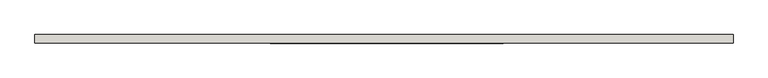
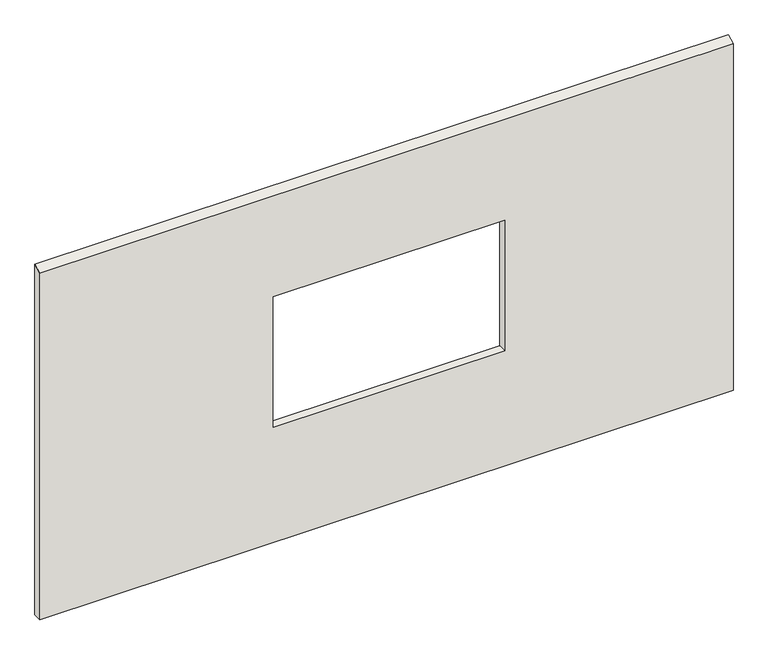
"""IFC4 building model written with IfcOpenShell, lengths in millimetres: wall geometry, 0_3d."""

import ifcopenshell
import ifcopenshell.guid

model = None  # the IFC model being written
_history = None  # IfcOwnerHistory: only IFC2X3 demands one
_inside = {}  # id of a spatial element -> (the spatial element, [elements in it])
_under = {}  # id of a project, library or spatial element -> (it, [spatial elements below it])
_declared = {}  # id of a project -> (the project, [libraries it declares])
_typed = {}  # id of a type object -> (the type object, [elements of that type])
_made_of = {}  # id of a material, layer set ... -> (it, [elements and type objects made of it])


def new_model(schema):
    """Start an empty IFC model of exactly this schema.

    Asked for "IFC4X3", IfcOpenShell would pick the latest addendum, in which some entities
    have other attributes; the version numbers below select the first issue.
    IFC2X3 requires an IfcOwnerHistory on every rooted entity: one is made here for all.
    """
    global model, _history
    if schema == "IFC4X3":
        model = ifcopenshell.file(schema_version=(4, 3, 0, 0))
    else:
        model = ifcopenshell.file(schema=schema)
    _inside.clear()
    _under.clear()
    _declared.clear()
    _typed.clear()
    _made_of.clear()
    _history = None
    if model.schema == "IFC2X3":
        org = make("IfcOrganization", Name="unknown")
        user = make(
            "IfcPersonAndOrganization",
            ThePerson=make("IfcPerson", FamilyName="unknown"),
            TheOrganization=org,
        )
        app = make(
            "IfcApplication",
            ApplicationDeveloper=org,
            Version="unknown",
            ApplicationFullName="unknown",
            ApplicationIdentifier="unknown",
        )
        _history = make(
            "IfcOwnerHistory",
            OwningUser=user,
            OwningApplication=app,
            ChangeAction="ADDED",
            CreationDate=0,
        )
    return model


def make(cls, **values):
    """One entity of the class cls with the attributes given. An attribute that is None is left unset."""
    return model.create_entity(
        cls, **{name: value for name, value in values.items() if value is not None}
    )


def rooted(cls, **values):
    """An entity with a GlobalId (a new one), such as an element, a storey or a relation."""
    return make(cls, GlobalId=ifcopenshell.guid.new(), OwnerHistory=_history, **values)


def si_unit(unit_type, name, prefix=None):
    """IfcSIUnit, for example si_unit("LENGTHUNIT", "METRE", prefix="MILLI")."""
    return make("IfcSIUnit", UnitType=unit_type, Prefix=prefix, Name=name)


def assignment(units):
    """IfcUnitAssignment: the units of a project."""
    return None if units is None else make("IfcUnitAssignment", Units=units)


def point(xyz):
    """IfcCartesianPoint."""
    return None if xyz is None else make("IfcCartesianPoint", Coordinates=xyz)


def direction(xyz):
    """IfcDirection."""
    return None if xyz is None else make("IfcDirection", DirectionRatios=xyz)


def frame(location, z_axis=None, x_axis=None):
    """IfcAxis2Placement3D, a coordinate frame: its origin and axes. An axis left out is left unset."""
    return make(
        "IfcAxis2Placement3D",
        Location=point(location),
        Axis=direction(z_axis),
        RefDirection=direction(x_axis),
    )


def origin():
    """The frame at (0, 0, 0) with its axes left unset."""
    return frame((0.0, 0.0, 0.0))


def place(relative_to, where):
    """IfcLocalPlacement: puts the frame where relative to a parent placement (None: the world)."""
    return make(
        "IfcLocalPlacement", PlacementRelTo=relative_to, RelativePlacement=where
    )


def context(
    kind, dimensions, precision=None, world=None, true_north=None, identifier=None
):
    """IfcGeometricRepresentationContext, for example the 3D "Model" context."""
    return make(
        "IfcGeometricRepresentationContext",
        ContextIdentifier=identifier,
        ContextType=kind,
        CoordinateSpaceDimension=dimensions,
        Precision=precision,
        WorldCoordinateSystem=world,
        TrueNorth=true_north,
    )


def project(units=None, contexts=None):
    """IfcProject with its units and contexts."""
    return rooted(
        "IfcProject",
        Name="project",
        RepresentationContexts=contexts,
        UnitsInContext=assignment(units),
    )


def spatial(cls, under=None, at=None, **own):
    """A site, building, storey or space (cls), placed at a placement, below another one or the project."""
    s = rooted(cls, ObjectPlacement=at, **own)
    if under is not None:
        _under.setdefault(under.id(), (under, []))[1].append(s)
    return s


def faces_of(points, faces, orient=None, outer=None):
    """IfcFace entities. A face is a list of loops; a loop is a list of indices into points, from 0.

    orient and outer hold one flag for each loop. By default every Orientation is true, the
    first loop of a face is its IfcFaceOuterBound and the others are IfcFaceBound.
    """
    made = []
    for i, loops in enumerate(faces):
        bounds = []
        for j, loop in enumerate(loops):
            is_outer = j == 0 if outer is None else outer[i][j]
            bounds.append(
                make(
                    "IfcFaceOuterBound" if is_outer else "IfcFaceBound",
                    Bound=make("IfcPolyLoop", Polygon=[points[k] for k in loop]),
                    Orientation=True if orient is None else orient[i][j],
                )
            )
        made.append(make("IfcFace", Bounds=bounds))
    return made


def faceted_brep(points, faces, orient=None, outer=None, voids=None):
    """IfcFacetedBrep: a solid bounded by flat faces; with voids (closed shells), ...WithVoids."""
    shared = [point(p) for p in points]
    hull = make("IfcClosedShell", CfsFaces=faces_of(shared, faces, orient, outer))
    if voids is None:
        return make("IfcFacetedBrep", Outer=hull)
    return make(
        "IfcFacetedBrepWithVoids",
        Outer=hull,
        Voids=[
            make(cls, CfsFaces=faces_of(shared, fs, o, b)) for cls, fs, o, b in voids
        ],
    )


def shape(context_of_items, identifier, shape_type, items):
    """IfcShapeRepresentation: the items that make up one representation, for example the "Body"."""
    return make(
        "IfcShapeRepresentation",
        ContextOfItems=context_of_items,
        RepresentationIdentifier=identifier,
        RepresentationType=shape_type,
        Items=items,
    )


def source(mapping_origin, context_of_items, identifier, shape_type, items):
    """IfcRepresentationMap: a shape defined once, which mapped items show again and again."""
    return make(
        "IfcRepresentationMap",
        MappingOrigin=mapping_origin,
        MappedRepresentation=shape(context_of_items, identifier, shape_type, items),
    )


def transform(
    local_origin,
    x_axis=None,
    y_axis=None,
    z_axis=None,
    scale=None,
    scale2=None,
    scale3=None,
    uniform=True,
):
    """IfcCartesianTransformationOperator3D, or its non-uniform kind. x_axis, y_axis, z_axis: its Axis1, 2, 3."""
    if uniform:
        return make(
            "IfcCartesianTransformationOperator3D",
            Axis1=direction(x_axis),
            Axis2=direction(y_axis),
            LocalOrigin=point(local_origin),
            Scale=scale,
            Axis3=direction(z_axis),
        )
    return make(
        "IfcCartesianTransformationOperator3DnonUniform",
        Axis1=direction(x_axis),
        Axis2=direction(y_axis),
        LocalOrigin=point(local_origin),
        Scale=scale,
        Axis3=direction(z_axis),
        Scale2=scale2,
        Scale3=scale3,
    )


def mapped(mapping_source, mapping_target):
    """IfcMappedItem: shows the shape of a source again, moved by a transform."""
    return make(
        "IfcMappedItem", MappingSource=mapping_source, MappingTarget=mapping_target
    )


def made_of(thing, what):
    """Note that an element or type object is made of a material, layer set ...; save() writes the relation."""
    if what is not None:
        _made_of.setdefault(what.id(), (what, []))[1].append(thing)
    return thing


def element(
    cls,
    number,
    at=None,
    inside=None,
    cuts=None,
    type_object=None,
    material=None,
    context=None,
    identifier="Body",
    shape_type=None,
    held_by="IfcProductDefinitionShape",
    body=None,
    shapes=None,
    **own,
):
    """One element of the class cls, such as IfcWall. Its Tag is "e" and its number.

    at: its placement. inside: the storey or other place that contains it. cuts: it is an
    opening in that element (IfcRelVoidsElement). A single representation is given by context,
    identifier, shape_type and body (its items); several are given by shapes. held_by: the class
    of the entity that holds the representations. save() writes the other relations.
    """
    e = rooted(cls, Tag="e%d" % number, ObjectPlacement=at, **own)
    if body is not None:
        shapes = [shape(context, identifier, shape_type, body)]
    if shapes is not None:
        e.Representation = make(held_by, Representations=shapes)
    if inside is not None:
        _inside.setdefault(inside.id(), (inside, []))[1].append(e)
    if cuts is not None:
        rooted(
            "IfcRelVoidsElement", RelatingBuildingElement=cuts, RelatedOpeningElement=e
        )
    if type_object is not None:
        _typed.setdefault(type_object.id(), (type_object, []))[1].append(e)
    return made_of(e, material)


def aggregate(whole, parts):
    """IfcRelAggregates: a whole, such as a stair, and the parts it consists of."""
    return rooted("IfcRelAggregates", RelatingObject=whole, RelatedObjects=parts)


def save(model, path):
    """Write the relations noted so far, then the file.

    IfcRelAggregates (storeys below a building ...), IfcRelContainedInSpatialStructure (elements
    in a storey), IfcRelDefinesByType, IfcRelAssociatesMaterial and IfcRelDeclares: one each for
    every whole, place, type object, material and project.
    """
    for whole, parts in _under.values():
        aggregate(whole, parts)
    for where, things in _inside.values():
        rooted(
            "IfcRelContainedInSpatialStructure",
            RelatedElements=things,
            RelatingStructure=where,
        )
    for kind, things in _typed.values():
        rooted("IfcRelDefinesByType", RelatedObjects=things, RelatingType=kind)
    for what, things in _made_of.values():
        rooted("IfcRelAssociatesMaterial", RelatedObjects=things, RelatingMaterial=what)
    for by, libraries in _declared.values():
        rooted("IfcRelDeclares", RelatingContext=by, RelatedDefinitions=libraries)
    model.write(path)


def wall_9d52c505(model_context):
    return source(origin(), model_context, "Body", "Brep", [
        faceted_brep([(1919.0, 70.0, 1000.0), (1919.0, 70.0, 2135.0), (1919.0, 0.0, 2135.0), (1919.0, 0.0, 1000.0), (3819.0, 70.0, 2135.0), (3819.0, 0.0, 2135.0), (3819.0, 70.0, 1000.0), (3819.0, 0.0, 1000.0), (0.0, 0.0, 3007.913011), (5694.0, 0.0, 3007.913011), (5694.0, 70.0, 3043.5797924), (0.0, 70.0, 3043.5797924), (5694.0, 0.0, 0.0), (5694.0, 70.0, 0.0), (0.0, 0.0, 0.0), (0.0, 70.0, 0.0)], [[[0, 1, 2, 3]], [[1, 4, 5, 2]], [[4, 6, 7, 5]], [[6, 0, 3, 7]], [[8, 9, 10, 11]], [[10, 9, 12, 13]], [[9, 8, 14, 12], [3, 2, 5, 7]], [[8, 11, 15, 14]], [[13, 15, 11, 10], [1, 0, 6, 4]], [[13, 12, 14, 15]]]),
    ])


if __name__ == "__main__":
    model = new_model("IFC4")
    model_context = context("Model", 3, world=origin())
    ifc_project = project(units=[si_unit("LENGTHUNIT", "METRE", prefix="MILLI")], contexts=[model_context])
    site = spatial("IfcSite", under=ifc_project)
    building = spatial("IfcBuilding", under=site)
    placement = place(None, origin())
    wall_shape = wall_9d52c505(model_context)
    element("IfcWall", 1, ObjectType="0_3d", at=placement, inside=building, context=model_context, shape_type="MappedRepresentation", body=[
        mapped(wall_shape, transform((0.0, 0.0, 0.0), x_axis=(1.0, 0.0, 0.0), y_axis=(0.0, 1.0, 0.0), z_axis=(0.0, 0.0, 1.0))),
    ])
    save(model, "model.ifc")

# Revit data of these elements
# Element 1 (IfcWall, "0_3d")
#   Materials on its faces: "Glass_Simple"
# Materials
#   "Glass_Simple": class "Unassigned", colour RGB 255 255 255, transparency 0.9
